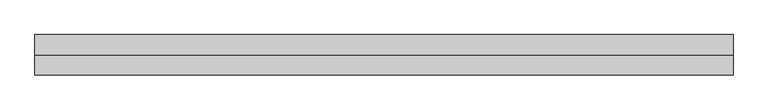
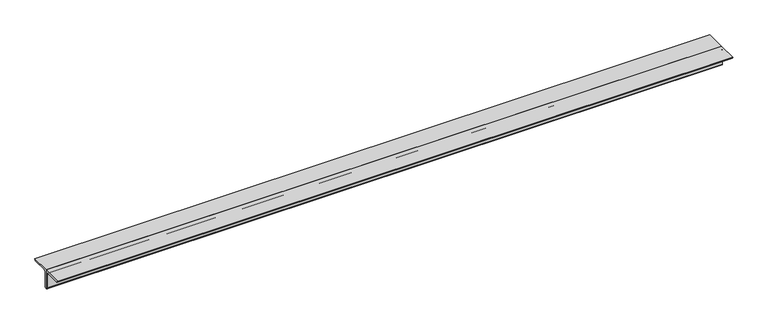
"""IFC4 building model written with IfcOpenShell, lengths in millimetres: beam geometry, 0123_Steel Framing_2Ls-KSD3502 : H_SB_AR_S03_2Ls-130x130x12_HBR4."""

import ifcopenshell
import ifcopenshell.guid

model = None  # the IFC model being written
_history = None  # IfcOwnerHistory: only IFC2X3 demands one
_inside = {}  # id of a spatial element -> (the spatial element, [elements in it])
_under = {}  # id of a project, library or spatial element -> (it, [spatial elements below it])
_declared = {}  # id of a project -> (the project, [libraries it declares])
_typed = {}  # id of a type object -> (the type object, [elements of that type])
_made_of = {}  # id of a material, layer set ... -> (it, [elements and type objects made of it])


def new_model(schema):
    """Start an empty IFC model of exactly this schema.

    Asked for "IFC4X3", IfcOpenShell would pick the latest addendum, in which some entities
    have other attributes; the version numbers below select the first issue.
    IFC2X3 requires an IfcOwnerHistory on every rooted entity: one is made here for all.
    """
    global model, _history
    if schema == "IFC4X3":
        model = ifcopenshell.file(schema_version=(4, 3, 0, 0))
    else:
        model = ifcopenshell.file(schema=schema)
    _inside.clear()
    _under.clear()
    _declared.clear()
    _typed.clear()
    _made_of.clear()
    _history = None
    if model.schema == "IFC2X3":
        org = make("IfcOrganization", Name="unknown")
        user = make(
            "IfcPersonAndOrganization",
            ThePerson=make("IfcPerson", FamilyName="unknown"),
            TheOrganization=org,
        )
        app = make(
            "IfcApplication",
            ApplicationDeveloper=org,
            Version="unknown",
            ApplicationFullName="unknown",
            ApplicationIdentifier="unknown",
        )
        _history = make(
            "IfcOwnerHistory",
            OwningUser=user,
            OwningApplication=app,
            ChangeAction="ADDED",
            CreationDate=0,
        )
    return model


def make(cls, **values):
    """One entity of the class cls with the attributes given. An attribute that is None is left unset."""
    return model.create_entity(
        cls, **{name: value for name, value in values.items() if value is not None}
    )


def rooted(cls, **values):
    """An entity with a GlobalId (a new one), such as an element, a storey or a relation."""
    return make(cls, GlobalId=ifcopenshell.guid.new(), OwnerHistory=_history, **values)


def si_unit(unit_type, name, prefix=None):
    """IfcSIUnit, for example si_unit("LENGTHUNIT", "METRE", prefix="MILLI")."""
    return make("IfcSIUnit", UnitType=unit_type, Prefix=prefix, Name=name)


def assignment(units):
    """IfcUnitAssignment: the units of a project."""
    return None if units is None else make("IfcUnitAssignment", Units=units)


def point(xyz):
    """IfcCartesianPoint."""
    return None if xyz is None else make("IfcCartesianPoint", Coordinates=xyz)


def direction(xyz):
    """IfcDirection."""
    return None if xyz is None else make("IfcDirection", DirectionRatios=xyz)


def frame(location, z_axis=None, x_axis=None):
    """IfcAxis2Placement3D, a coordinate frame: its origin and axes. An axis left out is left unset."""
    return make(
        "IfcAxis2Placement3D",
        Location=point(location),
        Axis=direction(z_axis),
        RefDirection=direction(x_axis),
    )


def frame_2d(location, x_axis=None):
    """IfcAxis2Placement2D, a coordinate frame in the plane: its origin and x axis."""
    return make(
        "IfcAxis2Placement2D", Location=point(location), RefDirection=direction(x_axis)
    )


def origin():
    """The frame at (0, 0, 0) with its axes left unset."""
    return frame((0.0, 0.0, 0.0))


def place(relative_to, where):
    """IfcLocalPlacement: puts the frame where relative to a parent placement (None: the world)."""
    return make(
        "IfcLocalPlacement", PlacementRelTo=relative_to, RelativePlacement=where
    )


def context(
    kind, dimensions, precision=None, world=None, true_north=None, identifier=None
):
    """IfcGeometricRepresentationContext, for example the 3D "Model" context."""
    return make(
        "IfcGeometricRepresentationContext",
        ContextIdentifier=identifier,
        ContextType=kind,
        CoordinateSpaceDimension=dimensions,
        Precision=precision,
        WorldCoordinateSystem=world,
        TrueNorth=true_north,
    )


def project(units=None, contexts=None):
    """IfcProject with its units and contexts."""
    return rooted(
        "IfcProject",
        Name="project",
        RepresentationContexts=contexts,
        UnitsInContext=assignment(units),
    )


def spatial(cls, under=None, at=None, **own):
    """A site, building, storey or space (cls), placed at a placement, below another one or the project."""
    s = rooted(cls, ObjectPlacement=at, **own)
    if under is not None:
        _under.setdefault(under.id(), (under, []))[1].append(s)
    return s


def polyline(points):
    """IfcPolyline through the points."""
    return make("IfcPolyline", Points=[point(p) for p in points])


def circle_curve(where, radius):
    """IfcCircle in the frame where."""
    return make("IfcCircle", Position=where, Radius=radius)


def trimmed(basis, trim1, trim2, sense, master):
    """IfcTrimmedCurve: the piece of a basis curve between two trims."""
    return make(
        "IfcTrimmedCurve",
        BasisCurve=basis,
        Trim1=trim1,
        Trim2=trim2,
        SenseAgreement=sense,
        MasterRepresentation=master,
    )


def segment(curve, same_sense, transition):
    """IfcCompositeCurveSegment."""
    return make(
        "IfcCompositeCurveSegment",
        Transition=transition,
        SameSense=same_sense,
        ParentCurve=curve,
    )


def composite_curve(segments, self_intersect=None):
    """IfcCompositeCurve: segments joined end to end."""
    return make("IfcCompositeCurve", Segments=segments, SelfIntersect=self_intersect)


def outline(outer, holes=None, kind="AREA"):
    """IfcArbitraryClosedProfileDef: a profile drawn as a closed curve; with holes, ...WithVoids."""
    if holes is None:
        return make("IfcArbitraryClosedProfileDef", ProfileType=kind, OuterCurve=outer)
    return make(
        "IfcArbitraryProfileDefWithVoids",
        ProfileType=kind,
        OuterCurve=outer,
        InnerCurves=holes,
    )


def extrude(swept, where, along, depth):
    """IfcExtrudedAreaSolid: the profile swept, set in the frame where, extruded along a direction by depth."""
    return make(
        "IfcExtrudedAreaSolid",
        SweptArea=swept,
        Position=where,
        ExtrudedDirection=direction(along),
        Depth=depth,
    )


def shape(context_of_items, identifier, shape_type, items):
    """IfcShapeRepresentation: the items that make up one representation, for example the "Body"."""
    return make(
        "IfcShapeRepresentation",
        ContextOfItems=context_of_items,
        RepresentationIdentifier=identifier,
        RepresentationType=shape_type,
        Items=items,
    )


def source(mapping_origin, context_of_items, identifier, shape_type, items):
    """IfcRepresentationMap: a shape defined once, which mapped items show again and again."""
    return make(
        "IfcRepresentationMap",
        MappingOrigin=mapping_origin,
        MappedRepresentation=shape(context_of_items, identifier, shape_type, items),
    )


def transform(
    local_origin,
    x_axis=None,
    y_axis=None,
    z_axis=None,
    scale=None,
    scale2=None,
    scale3=None,
    uniform=True,
):
    """IfcCartesianTransformationOperator3D, or its non-uniform kind. x_axis, y_axis, z_axis: its Axis1, 2, 3."""
    if uniform:
        return make(
            "IfcCartesianTransformationOperator3D",
            Axis1=direction(x_axis),
            Axis2=direction(y_axis),
            LocalOrigin=point(local_origin),
            Scale=scale,
            Axis3=direction(z_axis),
        )
    return make(
        "IfcCartesianTransformationOperator3DnonUniform",
        Axis1=direction(x_axis),
        Axis2=direction(y_axis),
        LocalOrigin=point(local_origin),
        Scale=scale,
        Axis3=direction(z_axis),
        Scale2=scale2,
        Scale3=scale3,
    )


def mapped(mapping_source, mapping_target):
    """IfcMappedItem: shows the shape of a source again, moved by a transform."""
    return make(
        "IfcMappedItem", MappingSource=mapping_source, MappingTarget=mapping_target
    )


def made_of(thing, what):
    """Note that an element or type object is made of a material, layer set ...; save() writes the relation."""
    if what is not None:
        _made_of.setdefault(what.id(), (what, []))[1].append(thing)
    return thing


def element(
    cls,
    number,
    at=None,
    inside=None,
    cuts=None,
    type_object=None,
    material=None,
    context=None,
    identifier="Body",
    shape_type=None,
    held_by="IfcProductDefinitionShape",
    body=None,
    shapes=None,
    **own,
):
    """One element of the class cls, such as IfcWall. Its Tag is "e" and its number.

    at: its placement. inside: the storey or other place that contains it. cuts: it is an
    opening in that element (IfcRelVoidsElement). A single representation is given by context,
    identifier, shape_type and body (its items); several are given by shapes. held_by: the class
    of the entity that holds the representations. save() writes the other relations.
    """
    e = rooted(cls, Tag="e%d" % number, ObjectPlacement=at, **own)
    if body is not None:
        shapes = [shape(context, identifier, shape_type, body)]
    if shapes is not None:
        e.Representation = make(held_by, Representations=shapes)
    if inside is not None:
        _inside.setdefault(inside.id(), (inside, []))[1].append(e)
    if cuts is not None:
        rooted(
            "IfcRelVoidsElement", RelatingBuildingElement=cuts, RelatedOpeningElement=e
        )
    if type_object is not None:
        _typed.setdefault(type_object.id(), (type_object, []))[1].append(e)
    return made_of(e, material)


def aggregate(whole, parts):
    """IfcRelAggregates: a whole, such as a stair, and the parts it consists of."""
    return rooted("IfcRelAggregates", RelatingObject=whole, RelatedObjects=parts)


def save(model, path):
    """Write the relations noted so far, then the file.

    IfcRelAggregates (storeys below a building ...), IfcRelContainedInSpatialStructure (elements
    in a storey), IfcRelDefinesByType, IfcRelAssociatesMaterial and IfcRelDeclares: one each for
    every whole, place, type object, material and project.
    """
    for whole, parts in _under.values():
        aggregate(whole, parts)
    for where, things in _inside.values():
        rooted(
            "IfcRelContainedInSpatialStructure",
            RelatedElements=things,
            RelatingStructure=where,
        )
    for kind, things in _typed.values():
        rooted("IfcRelDefinesByType", RelatedObjects=things, RelatingType=kind)
    for what, things in _made_of.values():
        rooted("IfcRelAssociatesMaterial", RelatedObjects=things, RelatingMaterial=what)
    for by, libraries in _declared.values():
        rooted("IfcRelDeclares", RelatingContext=by, RelatedDefinitions=libraries)
    model.write(path)


def beam_0d683159(model_context):
    return source(origin(), model_context, "Body", "SweptSolid", [
        extrude(outline(composite_curve([segment(polyline([(0.0, 36.4), (130.0, 36.4)]), True, "CONTINUOUS"), segment(trimmed(circle_curve(frame_2d((118.0, 36.4)), 12.0), [point((130.0, 36.4))], [point((118.0, 24.4))], False, "CARTESIAN"), True, "CONTINUOUS"), segment(polyline([(118.0, 24.4), (24.0, 24.4)]), True, "CONTINUOUS"), segment(trimmed(circle_curve(frame_2d((24.0, 12.4)), 12.0), [point((24.0, 24.4))], [point((12.0, 12.4))], True, "CARTESIAN"), True, "CONTINUOUS"), segment(polyline([(12.0, 12.4), (12.0, -81.6)]), True, "CONTINUOUS"), segment(trimmed(circle_curve(frame_2d((0.0, -81.6)), 12.0), [point((12.0, -81.6))], [point((0.0, -93.6))], False, "CARTESIAN"), True, "CONTINUOUS"), segment(polyline([(0.0, -93.6), (0.0, 36.4)]), True, "CONTINUOUS")], self_intersect=False)), frame((-2372.2356031, 0.0, 0.0), z_axis=(1.0, 0.0, 0.0), x_axis=(0.0, 1.0, 0.0)), (0.0, 0.0, 1.0), 4480.8559461),
        extrude(outline(composite_curve([segment(polyline([(0.0, 36.4), (0.0, -93.6)]), True, "CONTINUOUS"), segment(trimmed(circle_curve(frame_2d((0.0, -81.6)), 12.0), [point((0.0, -93.6))], [point((-12.0, -81.6))], False, "CARTESIAN"), True, "CONTINUOUS"), segment(polyline([(-12.0, -81.6), (-12.0, 12.4)]), True, "CONTINUOUS"), segment(trimmed(circle_curve(frame_2d((-24.0, 12.4)), 12.0), [point((-12.0, 12.4))], [point((-24.0, 24.4))], True, "CARTESIAN"), True, "CONTINUOUS"), segment(polyline([(-24.0, 24.4), (-118.0, 24.4)]), True, "CONTINUOUS"), segment(trimmed(circle_curve(frame_2d((-118.0, 36.4)), 12.0), [point((-118.0, 24.4))], [point((-130.0, 36.4))], False, "CARTESIAN"), True, "CONTINUOUS"), segment(polyline([(-130.0, 36.4), (0.0, 36.4)]), True, "CONTINUOUS")], self_intersect=False)), frame((-2372.2356031, 0.0, 0.0), z_axis=(1.0, 0.0, 0.0), x_axis=(0.0, 1.0, 0.0)), (0.0, 0.0, 1.0), 4480.8559461),
    ])


if __name__ == "__main__":
    model = new_model("IFC4")
    model_context = context("Model", 3, world=origin())
    ifc_project = project(units=[si_unit("LENGTHUNIT", "METRE", prefix="MILLI")], contexts=[model_context])
    site = spatial("IfcSite", under=ifc_project)
    building = spatial("IfcBuilding", under=site)
    placement = place(None, origin())
    beam_shape = beam_0d683159(model_context)
    element("IfcBeam", 1, ObjectType="0123_Steel Framing_2Ls-KSD3502 : H_SB_AR_S03_2Ls-130x130x12_HBR4", at=placement, inside=building, context=model_context, shape_type="MappedRepresentation", body=[
        mapped(beam_shape, transform((0.0, 0.0, 0.0), x_axis=(1.0, 0.0, 0.0), y_axis=(0.0, 1.0, 0.0), z_axis=(0.0, 0.0, 1.0))),
    ])
    save(model, "model.ifc")

# Revit data of these elements
# Type "0123_Steel Framing_2Ls-KSD3502 : H_SB_AR_S03_2Ls-130x130x12_HBR4"
#   Assembly Code = "B10"
#   Legs = "SLBB"
#   W = 8.97
#   Perimeter = 1.04 m²/m
#   Nominal Weight = 46.80 kgf/m
#   Length [instance default] = 1000 mm
#   Space = 0 mm
#   b = 130 mm
#   d = 130 mm
#   t = 12 mm
#   y = 36.4 mm
#   A = 0.005952 m²
#   Structural Material [instance default] = Steel ASTM A36
# Element 1 (IfcBeam, "0123_Steel Framing_2Ls-KSD3502 : H_SB_AR_S03_2Ls-130x130x12_HBR4")
#   Structural Material = Steel, 45-345
#   Materials on its faces: "Steel, 45-345"
# Materials
#   "Steel ASTM A36": class "Metal", colour RGB 199 199 199, transparency 0, Description = "Structural steel, ASTM A36 Grade B, mill finish", Cost = 0
#   "Steel, 45-345": class "Metal", colour RGB 189 187 185, transparency 0, Description = "Steel 345 MPa", Cost = 0
